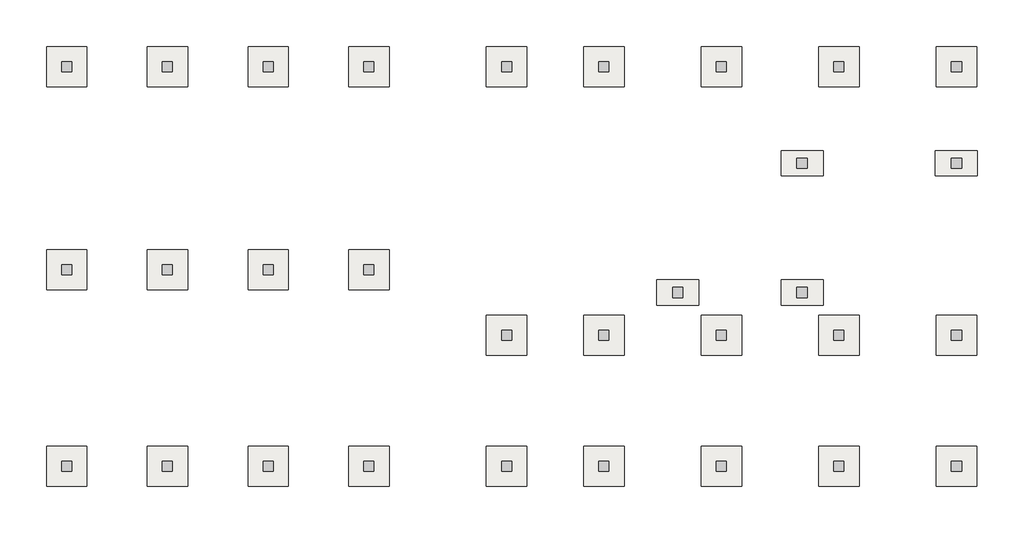
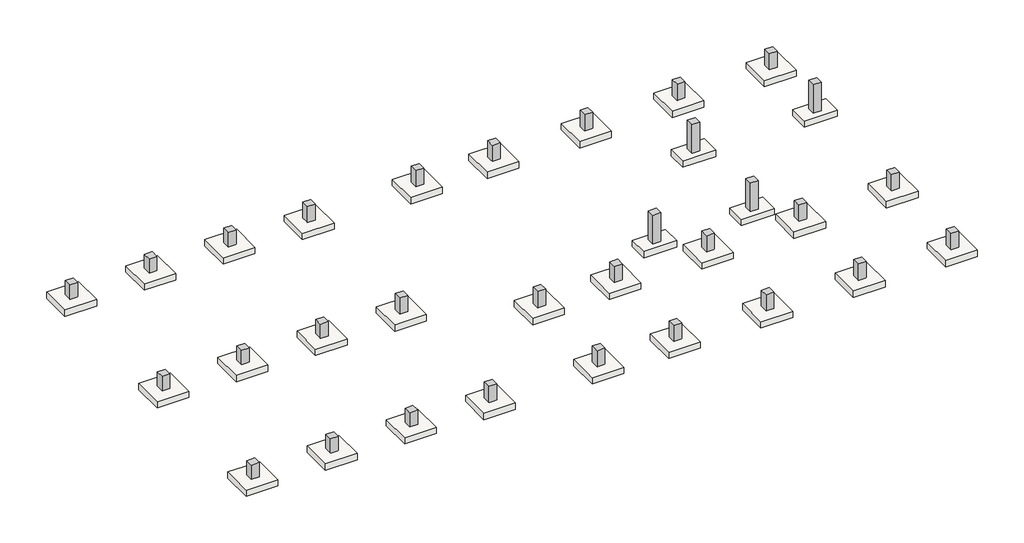
# Not in any storey: 31 columns, 31 slabs.
"""IFC4 building model written with IfcOpenShell, lengths in millimetres."""

import ifcopenshell
import ifcopenshell.guid

model = None  # the IFC model being written
_history = None  # IfcOwnerHistory: only IFC2X3 demands one
_inside = {}  # id of a spatial element -> (the spatial element, [elements in it])
_under = {}  # id of a project, library or spatial element -> (it, [spatial elements below it])
_declared = {}  # id of a project -> (the project, [libraries it declares])
_typed = {}  # id of a type object -> (the type object, [elements of that type])
_made_of = {}  # id of a material, layer set ... -> (it, [elements and type objects made of it])


def new_model(schema):
    """Start an empty IFC model of exactly this schema.

    Asked for "IFC4X3", IfcOpenShell would pick the latest addendum, in which some entities
    have other attributes; the version numbers below select the first issue.
    IFC2X3 requires an IfcOwnerHistory on every rooted entity: one is made here for all.
    """
    global model, _history
    if schema == "IFC4X3":
        model = ifcopenshell.file(schema_version=(4, 3, 0, 0))
    else:
        model = ifcopenshell.file(schema=schema)
    _inside.clear()
    _under.clear()
    _declared.clear()
    _typed.clear()
    _made_of.clear()
    _history = None
    if model.schema == "IFC2X3":
        org = make("IfcOrganization", Name="unknown")
        user = make(
            "IfcPersonAndOrganization",
            ThePerson=make("IfcPerson", FamilyName="unknown"),
            TheOrganization=org,
        )
        app = make(
            "IfcApplication",
            ApplicationDeveloper=org,
            Version="unknown",
            ApplicationFullName="unknown",
            ApplicationIdentifier="unknown",
        )
        _history = make(
            "IfcOwnerHistory",
            OwningUser=user,
            OwningApplication=app,
            ChangeAction="ADDED",
            CreationDate=0,
        )
    return model


def make(cls, **values):
    """One entity of the class cls with the attributes given. An attribute that is None is left unset."""
    return model.create_entity(
        cls, **{name: value for name, value in values.items() if value is not None}
    )


def rooted(cls, **values):
    """An entity with a GlobalId (a new one), such as an element, a storey or a relation."""
    return make(cls, GlobalId=ifcopenshell.guid.new(), OwnerHistory=_history, **values)


def si_unit(unit_type, name, prefix=None):
    """IfcSIUnit, for example si_unit("LENGTHUNIT", "METRE", prefix="MILLI")."""
    return make("IfcSIUnit", UnitType=unit_type, Prefix=prefix, Name=name)


def assignment(units):
    """IfcUnitAssignment: the units of a project."""
    return None if units is None else make("IfcUnitAssignment", Units=units)


def point(xyz):
    """IfcCartesianPoint."""
    return None if xyz is None else make("IfcCartesianPoint", Coordinates=xyz)


def direction(xyz):
    """IfcDirection."""
    return None if xyz is None else make("IfcDirection", DirectionRatios=xyz)


def frame(location, z_axis=None, x_axis=None):
    """IfcAxis2Placement3D, a coordinate frame: its origin and axes. An axis left out is left unset."""
    return make(
        "IfcAxis2Placement3D",
        Location=point(location),
        Axis=direction(z_axis),
        RefDirection=direction(x_axis),
    )


def origin():
    """The frame at (0, 0, 0) with its axes left unset."""
    return frame((0.0, 0.0, 0.0))


def place(relative_to, where):
    """IfcLocalPlacement: puts the frame where relative to a parent placement (None: the world)."""
    return make(
        "IfcLocalPlacement", PlacementRelTo=relative_to, RelativePlacement=where
    )


def context(
    kind, dimensions, precision=None, world=None, true_north=None, identifier=None
):
    """IfcGeometricRepresentationContext, for example the 3D "Model" context."""
    return make(
        "IfcGeometricRepresentationContext",
        ContextIdentifier=identifier,
        ContextType=kind,
        CoordinateSpaceDimension=dimensions,
        Precision=precision,
        WorldCoordinateSystem=world,
        TrueNorth=true_north,
    )


def project(units=None, contexts=None):
    """IfcProject with its units and contexts."""
    return rooted(
        "IfcProject",
        Name="project",
        RepresentationContexts=contexts,
        UnitsInContext=assignment(units),
    )


def spatial(cls, under=None, at=None, **own):
    """A site, building, storey or space (cls), placed at a placement, below another one or the project."""
    s = rooted(cls, ObjectPlacement=at, **own)
    if under is not None:
        _under.setdefault(under.id(), (under, []))[1].append(s)
    return s


def polyline(points):
    """IfcPolyline through the points."""
    return make("IfcPolyline", Points=[point(p) for p in points])


def outline(outer, holes=None, kind="AREA"):
    """IfcArbitraryClosedProfileDef: a profile drawn as a closed curve; with holes, ...WithVoids."""
    if holes is None:
        return make("IfcArbitraryClosedProfileDef", ProfileType=kind, OuterCurve=outer)
    return make(
        "IfcArbitraryProfileDefWithVoids",
        ProfileType=kind,
        OuterCurve=outer,
        InnerCurves=holes,
    )


def extrude(swept, where, along, depth):
    """IfcExtrudedAreaSolid: the profile swept, set in the frame where, extruded along a direction by depth."""
    return make(
        "IfcExtrudedAreaSolid",
        SweptArea=swept,
        Position=where,
        ExtrudedDirection=direction(along),
        Depth=depth,
    )


def shape(context_of_items, identifier, shape_type, items):
    """IfcShapeRepresentation: the items that make up one representation, for example the "Body"."""
    return make(
        "IfcShapeRepresentation",
        ContextOfItems=context_of_items,
        RepresentationIdentifier=identifier,
        RepresentationType=shape_type,
        Items=items,
    )


def source(mapping_origin, context_of_items, identifier, shape_type, items):
    """IfcRepresentationMap: a shape defined once, which mapped items show again and again."""
    return make(
        "IfcRepresentationMap",
        MappingOrigin=mapping_origin,
        MappedRepresentation=shape(context_of_items, identifier, shape_type, items),
    )


def transform(
    local_origin,
    x_axis=None,
    y_axis=None,
    z_axis=None,
    scale=None,
    scale2=None,
    scale3=None,
    uniform=True,
):
    """IfcCartesianTransformationOperator3D, or its non-uniform kind. x_axis, y_axis, z_axis: its Axis1, 2, 3."""
    if uniform:
        return make(
            "IfcCartesianTransformationOperator3D",
            Axis1=direction(x_axis),
            Axis2=direction(y_axis),
            LocalOrigin=point(local_origin),
            Scale=scale,
            Axis3=direction(z_axis),
        )
    return make(
        "IfcCartesianTransformationOperator3DnonUniform",
        Axis1=direction(x_axis),
        Axis2=direction(y_axis),
        LocalOrigin=point(local_origin),
        Scale=scale,
        Axis3=direction(z_axis),
        Scale2=scale2,
        Scale3=scale3,
    )


def mapped(mapping_source, mapping_target):
    """IfcMappedItem: shows the shape of a source again, moved by a transform."""
    return make(
        "IfcMappedItem", MappingSource=mapping_source, MappingTarget=mapping_target
    )


def made_of(thing, what):
    """Note that an element or type object is made of a material, layer set ...; save() writes the relation."""
    if what is not None:
        _made_of.setdefault(what.id(), (what, []))[1].append(thing)
    return thing


def element(
    cls,
    number,
    at=None,
    inside=None,
    cuts=None,
    type_object=None,
    material=None,
    context=None,
    identifier="Body",
    shape_type=None,
    held_by="IfcProductDefinitionShape",
    body=None,
    shapes=None,
    **own,
):
    """One element of the class cls, such as IfcWall. Its Tag is "e" and its number.

    at: its placement. inside: the storey or other place that contains it. cuts: it is an
    opening in that element (IfcRelVoidsElement). A single representation is given by context,
    identifier, shape_type and body (its items); several are given by shapes. held_by: the class
    of the entity that holds the representations. save() writes the other relations.
    """
    e = rooted(cls, Tag="e%d" % number, ObjectPlacement=at, **own)
    if body is not None:
        shapes = [shape(context, identifier, shape_type, body)]
    if shapes is not None:
        e.Representation = make(held_by, Representations=shapes)
    if inside is not None:
        _inside.setdefault(inside.id(), (inside, []))[1].append(e)
    if cuts is not None:
        rooted(
            "IfcRelVoidsElement", RelatingBuildingElement=cuts, RelatedOpeningElement=e
        )
    if type_object is not None:
        _typed.setdefault(type_object.id(), (type_object, []))[1].append(e)
    return made_of(e, material)


def aggregate(whole, parts):
    """IfcRelAggregates: a whole, such as a stair, and the parts it consists of."""
    return rooted("IfcRelAggregates", RelatingObject=whole, RelatedObjects=parts)


def save(model, path):
    """Write the relations noted so far, then the file.

    IfcRelAggregates (storeys below a building ...), IfcRelContainedInSpatialStructure (elements
    in a storey), IfcRelDefinesByType, IfcRelAssociatesMaterial and IfcRelDeclares: one each for
    every whole, place, type object, material and project.
    """
    for whole, parts in _under.values():
        aggregate(whole, parts)
    for where, things in _inside.values():
        rooted(
            "IfcRelContainedInSpatialStructure",
            RelatedElements=things,
            RelatingStructure=where,
        )
    for kind, things in _typed.values():
        rooted("IfcRelDefinesByType", RelatedObjects=things, RelatingType=kind)
    for what, things in _made_of.values():
        rooted("IfcRelAssociatesMaterial", RelatedObjects=things, RelatingMaterial=what)
    for by, libraries in _declared.values():
        rooted("IfcRelDeclares", RelatingContext=by, RelatedDefinitions=libraries)
    model.write(path)


def ft211_footing_rectangular_r1_5fe39465(model_context):
    return source(origin(), model_context, "Body", "SweptSolid", [
        extrude(outline(polyline([(1200.0, 1200.0), (1200.0, -1200.0), (-1200.0, -1200.0), (-1200.0, 1200.0), (1200.0, 1200.0)])), frame((0.0, 0.0, -500.0), z_axis=(0.0, 0.0, 1.0), x_axis=(1.0, 0.0, 0.0)), (0.0, 0.0, 1.0), 500.0),
    ])


def ft211_footing_rectangular_r1_907a7f09(model_context):
    return source(origin(), model_context, "Body", "SweptSolid", [
        extrude(outline(polyline([(1250.0, 750.0), (1250.0, -750.0), (-1250.0, -750.0), (-1250.0, 750.0), (1250.0, 750.0)])), frame((0.0, 0.0, -500.0), z_axis=(0.0, 0.0, 1.0), x_axis=(1.0, 0.0, 0.0)), (0.0, 0.0, 1.0), 500.0),
    ])


model = new_model("IFC4")

# Units and contexts
model_context = context("Model", 3, world=origin())
ifc_project = project(units=[si_unit("LENGTHUNIT", "METRE", prefix="MILLI")], contexts=[model_context])

# Site, building
site = spatial("IfcSite", under=ifc_project)
building = spatial("IfcBuilding", under=site)

# Columns
placement = place(None, origin())
element("IfcColumn", 1, ObjectType="RC_Column_Rectangular : H_SC_ACC_UG PED_W600xL600", at=placement, inside=building, context=model_context, shape_type="SweptSolid", body=[
    extrude(outline(polyline([(224.7, 12616.5208589), (224.7, 12016.5208589), (-375.3, 12016.5208589), (-375.3, 12616.5208589), (224.7, 12616.5208589)])), frame((0.0, 0.0, -1000.0), z_axis=(0.0, 0.0, 1.0), x_axis=(1.0, 0.0, 0.0)), (0.0, 0.0, 1.0), 1150.0),
])
element("IfcColumn", 2, ObjectType="RC_Column_Rectangular : H_SC_ACC_UG PED_W600xL600", at=placement, inside=building, context=model_context, shape_type="SweptSolid", body=[
    extrude(outline(polyline([(6224.7, 12616.5208589), (6224.7, 12016.5208589), (5624.7, 12016.5208589), (5624.7, 12616.5208589), (6224.7, 12616.5208589)])), frame((0.0, 0.0, -1000.0), z_axis=(0.0, 0.0, 1.0), x_axis=(1.0, 0.0, 0.0)), (0.0, 0.0, 1.0), 1150.0),
])
element("IfcColumn", 3, ObjectType="RC_Column_Rectangular : H_SC_ACC_UG PED_W600xL600", at=placement, inside=building, context=model_context, shape_type="SweptSolid", body=[
    extrude(outline(polyline([(12224.7, 12616.5208589), (12224.7, 12016.5208589), (11624.7, 12016.5208589), (11624.7, 12616.5208589), (12224.7, 12616.5208589)])), frame((0.0, 0.0, -1000.0), z_axis=(0.0, 0.0, 1.0), x_axis=(1.0, 0.0, 0.0)), (0.0, 0.0, 1.0), 1150.0),
])
element("IfcColumn", 4, ObjectType="RC_Column_Rectangular : H_SC_ACC_UG PED_W600xL600", at=placement, inside=building, context=model_context, shape_type="SweptSolid", body=[
    extrude(outline(polyline([(18224.7, 12616.5208589), (18224.7, 12016.5208589), (17624.7, 12016.5208589), (17624.7, 12616.5208589), (18224.7, 12616.5208589)])), frame((0.0, 0.0, -1150.0), z_axis=(0.0, 0.0, 1.0), x_axis=(1.0, 0.0, 0.0)), (0.0, 0.0, 1.0), 1300.0),
])
element("IfcColumn", 5, ObjectType="RC_Column_Rectangular : H_SC_ACC_UG PED_W600xL600", at=placement, inside=building, context=model_context, shape_type="SweptSolid", body=[
    extrude(outline(polyline([(224.7, 24716.5208589), (224.7, 24116.5208589), (-375.3, 24116.5208589), (-375.3, 24716.5208589), (224.7, 24716.5208589)])), frame((0.0, 0.0, -1000.0), z_axis=(0.0, 0.0, 1.0), x_axis=(1.0, 0.0, 0.0)), (0.0, 0.0, 1.0), 1150.0),
])
element("IfcColumn", 6, ObjectType="RC_Column_Rectangular : H_SC_ACC_UG PED_W600xL600", at=placement, inside=building, context=model_context, shape_type="SweptSolid", body=[
    extrude(outline(polyline([(6224.7, 24716.5208589), (6224.7, 24116.5208589), (5624.7, 24116.5208589), (5624.7, 24716.5208589), (6224.7, 24716.5208589)])), frame((0.0, 0.0, -1000.0), z_axis=(0.0, 0.0, 1.0), x_axis=(1.0, 0.0, 0.0)), (0.0, 0.0, 1.0), 1150.0),
])
element("IfcColumn", 7, ObjectType="RC_Column_Rectangular : H_SC_ACC_UG PED_W600xL600", at=placement, inside=building, context=model_context, shape_type="SweptSolid", body=[
    extrude(outline(polyline([(12224.7, 24716.5208589), (12224.7, 24116.5208589), (11624.7, 24116.5208589), (11624.7, 24716.5208589), (12224.7, 24716.5208589)])), frame((0.0, 0.0, -1000.0), z_axis=(0.0, 0.0, 1.0), x_axis=(1.0, 0.0, 0.0)), (0.0, 0.0, 1.0), 1150.0),
])
element("IfcColumn", 8, ObjectType="RC_Column_Rectangular : H_SC_ACC_UG PED_W600xL600", at=placement, inside=building, context=model_context, shape_type="SweptSolid", body=[
    extrude(outline(polyline([(18224.7, 24716.5208589), (18224.7, 24116.5208589), (17624.7, 24116.5208589), (17624.7, 24716.5208589), (18224.7, 24716.5208589)])), frame((0.0, 0.0, -1150.0), z_axis=(0.0, 0.0, 1.0), x_axis=(1.0, 0.0, 0.0)), (0.0, 0.0, 1.0), 1300.0),
])
element("IfcColumn", 9, ObjectType="RC_Column_Rectangular : H_SC_ACC_UG PED_W600xL600", at=placement, inside=building, context=model_context, shape_type="SweptSolid", body=[
    extrude(outline(polyline([(26424.7, 24716.5208589), (26424.7, 24116.5208589), (25824.7, 24116.5208589), (25824.7, 24716.5208589), (26424.7, 24716.5208589)])), frame((0.0, 0.0, -1150.0), z_axis=(0.0, 0.0, 1.0), x_axis=(1.0, 0.0, 0.0)), (0.0, 0.0, 1.0), 1300.0),
])
element("IfcColumn", 10, ObjectType="RC_Column_Rectangular : H_SC_ACC_UG PED_W600xL600", at=placement, inside=building, context=model_context, shape_type="SweptSolid", body=[
    extrude(outline(polyline([(32224.7, 24716.5208589), (32224.7, 24116.5208589), (31624.7, 24116.5208589), (31624.7, 24716.5208589), (32224.7, 24716.5208589)])), frame((0.0, 0.0, -1150.0), z_axis=(0.0, 0.0, 1.0), x_axis=(1.0, 0.0, 0.0)), (0.0, 0.0, 1.0), 1300.0),
])
element("IfcColumn", 11, ObjectType="RC_Column_Rectangular : H_SC_ACC_UG PED_W600xL600", at=placement, inside=building, context=model_context, shape_type="SweptSolid", body=[
    extrude(outline(polyline([(39224.7, 24716.5208589), (39224.7, 24116.5208589), (38624.7, 24116.5208589), (38624.7, 24716.5208589), (39224.7, 24716.5208589)])), frame((0.0, 0.0, -1150.0), z_axis=(0.0, 0.0, 1.0), x_axis=(1.0, 0.0, 0.0)), (0.0, 0.0, 1.0), 1300.0),
])
element("IfcColumn", 12, ObjectType="RC_Column_Rectangular : H_SC_ACC_UG PED_W600xL600", at=placement, inside=building, context=model_context, shape_type="SweptSolid", body=[
    extrude(outline(polyline([(46224.7, 24716.5208589), (46224.7, 24116.5208589), (45624.7, 24116.5208589), (45624.7, 24716.5208589), (46224.7, 24716.5208589)])), frame((0.0, 0.0, -1150.0), z_axis=(0.0, 0.0, 1.0), x_axis=(1.0, 0.0, 0.0)), (0.0, 0.0, 1.0), 1300.0),
])
element("IfcColumn", 13, ObjectType="RC_Column_Rectangular : H_SC_ACC_UG PED_W600xL600", at=placement, inside=building, context=model_context, shape_type="SweptSolid", body=[
    extrude(outline(polyline([(53224.7, 24716.5208589), (53224.7, 24116.5208589), (52624.7, 24116.5208589), (52624.7, 24716.5208589), (53224.7, 24716.5208589)])), frame((0.0, 0.0, -1150.0), z_axis=(0.0, 0.0, 1.0), x_axis=(1.0, 0.0, 0.0)), (0.0, 0.0, 1.0), 1300.0),
])
element("IfcColumn", 14, ObjectType="RC_Column_Rectangular : H_SC_ACC_UG PED_W600xL600", at=placement, inside=building, context=model_context, shape_type="SweptSolid", body=[
    extrude(outline(polyline([(26424.7, 8716.5208589), (26424.7, 8116.5208589), (25824.7, 8116.5208589), (25824.7, 8716.5208589), (26424.7, 8716.5208589)])), frame((0.0, 0.0, -1150.0), z_axis=(0.0, 0.0, 1.0), x_axis=(1.0, 0.0, 0.0)), (0.0, 0.0, 1.0), 1300.0),
])
element("IfcColumn", 15, ObjectType="RC_Column_Rectangular : H_SC_ACC_UG PED_W600xL600", at=placement, inside=building, context=model_context, shape_type="SweptSolid", body=[
    extrude(outline(polyline([(32224.7, 8716.5208589), (32224.7, 8116.5208589), (31624.7, 8116.5208589), (31624.7, 8716.5208589), (32224.7, 8716.5208589)])), frame((0.0, 0.0, -1150.0), z_axis=(0.0, 0.0, 1.0), x_axis=(1.0, 0.0, 0.0)), (0.0, 0.0, 1.0), 1300.0),
])
element("IfcColumn", 16, ObjectType="RC_Column_Rectangular : H_SC_ACC_UG PED_W600xL600", at=placement, inside=building, context=model_context, shape_type="SweptSolid", body=[
    extrude(outline(polyline([(39224.7, 8716.5208589), (39224.7, 8116.5208589), (38624.7, 8116.5208589), (38624.7, 8716.5208589), (39224.7, 8716.5208589)])), frame((0.0, 0.0, -1150.0), z_axis=(0.0, 0.0, 1.0), x_axis=(1.0, 0.0, 0.0)), (0.0, 0.0, 1.0), 1300.0),
])
element("IfcColumn", 17, ObjectType="RC_Column_Rectangular : H_SC_ACC_UG PED_W600xL600", at=placement, inside=building, context=model_context, shape_type="SweptSolid", body=[
    extrude(outline(polyline([(46224.7, 8716.5208589), (46224.7, 8116.5208589), (45624.7, 8116.5208589), (45624.7, 8716.5208589), (46224.7, 8716.5208589)])), frame((0.0, 0.0, -1150.0), z_axis=(0.0, 0.0, 1.0), x_axis=(1.0, 0.0, 0.0)), (0.0, 0.0, 1.0), 1300.0),
])
element("IfcColumn", 18, ObjectType="RC_Column_Rectangular : H_SC_ACC_UG PED_W600xL600", at=placement, inside=building, context=model_context, shape_type="SweptSolid", body=[
    extrude(outline(polyline([(53224.7, 8716.5208589), (53224.7, 8116.5208589), (52624.7, 8116.5208589), (52624.7, 8716.5208589), (53224.7, 8716.5208589)])), frame((0.0, 0.0, -1150.0), z_axis=(0.0, 0.0, 1.0), x_axis=(1.0, 0.0, 0.0)), (0.0, 0.0, 1.0), 1300.0),
])
element("IfcColumn", 19, ObjectType="RC_Column_Rectangular : H_SC_ACC_UG PED_W600xL600", at=placement, inside=building, context=model_context, shape_type="SweptSolid", body=[
    extrude(outline(polyline([(224.7, 916.5208589), (224.7, 316.5208589), (-375.3, 316.5208589), (-375.3, 916.5208589), (224.7, 916.5208589)])), frame((0.0, 0.0, -1000.0), z_axis=(0.0, 0.0, 1.0), x_axis=(1.0, 0.0, 0.0)), (0.0, 0.0, 1.0), 1150.0),
])
element("IfcColumn", 20, ObjectType="RC_Column_Rectangular : H_SC_ACC_UG PED_W600xL600", at=placement, inside=building, context=model_context, shape_type="SweptSolid", body=[
    extrude(outline(polyline([(6224.7, 916.5208589), (6224.7, 316.5208589), (5624.7, 316.5208589), (5624.7, 916.5208589), (6224.7, 916.5208589)])), frame((0.0, 0.0, -1000.0), z_axis=(0.0, 0.0, 1.0), x_axis=(1.0, 0.0, 0.0)), (0.0, 0.0, 1.0), 1150.0),
])
element("IfcColumn", 21, ObjectType="RC_Column_Rectangular : H_SC_ACC_UG PED_W600xL600", at=placement, inside=building, context=model_context, shape_type="SweptSolid", body=[
    extrude(outline(polyline([(12224.7, 916.5208589), (12224.7, 316.5208589), (11624.7, 316.5208589), (11624.7, 916.5208589), (12224.7, 916.5208589)])), frame((0.0, 0.0, -1000.0), z_axis=(0.0, 0.0, 1.0), x_axis=(1.0, 0.0, 0.0)), (0.0, 0.0, 1.0), 1150.0),
])
element("IfcColumn", 22, ObjectType="RC_Column_Rectangular : H_SC_ACC_UG PED_W600xL600", at=placement, inside=building, context=model_context, shape_type="SweptSolid", body=[
    extrude(outline(polyline([(18224.7, 916.5208589), (18224.7, 316.5208589), (17624.7, 316.5208589), (17624.7, 916.5208589), (18224.7, 916.5208589)])), frame((0.0, 0.0, -1150.0), z_axis=(0.0, 0.0, 1.0), x_axis=(1.0, 0.0, 0.0)), (0.0, 0.0, 1.0), 1300.0),
])
element("IfcColumn", 23, ObjectType="RC_Column_Rectangular : H_SC_ACC_UG PED_W600xL600", at=placement, inside=building, context=model_context, shape_type="SweptSolid", body=[
    extrude(outline(polyline([(26424.7, 916.5208589), (26424.7, 316.5208589), (25824.7, 316.5208589), (25824.7, 916.5208589), (26424.7, 916.5208589)])), frame((0.0, 0.0, -1150.0), z_axis=(0.0, 0.0, 1.0), x_axis=(1.0, 0.0, 0.0)), (0.0, 0.0, 1.0), 1300.0),
])
element("IfcColumn", 24, ObjectType="RC_Column_Rectangular : H_SC_ACC_UG PED_W600xL600", at=placement, inside=building, context=model_context, shape_type="SweptSolid", body=[
    extrude(outline(polyline([(32224.7, 916.5208589), (32224.7, 316.5208589), (31624.7, 316.5208589), (31624.7, 916.5208589), (32224.7, 916.5208589)])), frame((0.0, 0.0, -1150.0), z_axis=(0.0, 0.0, 1.0), x_axis=(1.0, 0.0, 0.0)), (0.0, 0.0, 1.0), 1300.0),
])
element("IfcColumn", 25, ObjectType="RC_Column_Rectangular : H_SC_ACC_UG PED_W600xL600", at=placement, inside=building, context=model_context, shape_type="SweptSolid", body=[
    extrude(outline(polyline([(39224.7, 916.5208589), (39224.7, 316.5208589), (38624.7, 316.5208589), (38624.7, 916.5208589), (39224.7, 916.5208589)])), frame((0.0, 0.0, -1150.0), z_axis=(0.0, 0.0, 1.0), x_axis=(1.0, 0.0, 0.0)), (0.0, 0.0, 1.0), 1300.0),
])
element("IfcColumn", 26, ObjectType="RC_Column_Rectangular : H_SC_ACC_UG PED_W600xL600", at=placement, inside=building, context=model_context, shape_type="SweptSolid", body=[
    extrude(outline(polyline([(46224.7, 916.5208589), (46224.7, 316.5208589), (45624.7, 316.5208589), (45624.7, 916.5208589), (46224.7, 916.5208589)])), frame((0.0, 0.0, -1150.0), z_axis=(0.0, 0.0, 1.0), x_axis=(1.0, 0.0, 0.0)), (0.0, 0.0, 1.0), 1300.0),
])
element("IfcColumn", 27, ObjectType="RC_Column_Rectangular : H_SC_ACC_UG PED_W600xL600", at=placement, inside=building, context=model_context, shape_type="SweptSolid", body=[
    extrude(outline(polyline([(53224.7, 916.5208589), (53224.7, 316.5208589), (52624.7, 316.5208589), (52624.7, 916.5208589), (53224.7, 916.5208589)])), frame((0.0, 0.0, -1150.0), z_axis=(0.0, 0.0, 1.0), x_axis=(1.0, 0.0, 0.0)), (0.0, 0.0, 1.0), 1300.0),
])
element("IfcColumn", 28, ObjectType="RC_Column_Rectangular : H_SC_ACC_UG PED_W600xL600", at=placement, inside=building, context=model_context, shape_type="SweptSolid", body=[
    extrude(outline(polyline([(36624.7, 11266.5208589), (36624.7, 10666.5208589), (36024.7, 10666.5208589), (36024.7, 11266.5208589), (36624.7, 11266.5208589)])), frame((0.0, 0.0, -1150.0), z_axis=(0.0, 0.0, 1.0), x_axis=(1.0, 0.0, 0.0)), (0.0, 0.0, 1.0), 2300.0),
])
element("IfcColumn", 29, ObjectType="RC_Column_Rectangular : H_SC_ACC_UG PED_W600xL600", at=placement, inside=building, context=model_context, shape_type="SweptSolid", body=[
    extrude(outline(polyline([(44024.7, 11266.5208589), (44024.7, 10666.5208589), (43424.7, 10666.5208589), (43424.7, 11266.5208589), (44024.7, 11266.5208589)])), frame((0.0, 0.0, -1150.0), z_axis=(0.0, 0.0, 1.0), x_axis=(1.0, 0.0, 0.0)), (0.0, 0.0, 1.0), 2300.0),
])
element("IfcColumn", 30, ObjectType="RC_Column_Rectangular : H_SC_ACC_UG PED_W600xL600", at=placement, inside=building, context=model_context, shape_type="SweptSolid", body=[
    extrude(outline(polyline([(44024.7, 18966.5208589), (44024.7, 18366.5208589), (43424.7, 18366.5208589), (43424.7, 18966.5208589), (44024.7, 18966.5208589)])), frame((0.0, 0.0, -1150.0), z_axis=(0.0, 0.0, 1.0), x_axis=(1.0, 0.0, 0.0)), (0.0, 0.0, 1.0), 2300.0),
])
element("IfcColumn", 31, ObjectType="RC_Column_Rectangular : H_SC_ACC_UG PED_W600xL600", at=placement, inside=building, context=model_context, shape_type="SweptSolid", body=[
    extrude(outline(polyline([(53224.7, 18966.5208589), (53224.7, 18366.5208589), (52624.7, 18366.5208589), (52624.7, 18966.5208589), (53224.7, 18966.5208589)])), frame((0.0, 0.0, -1150.0), z_axis=(0.0, 0.0, 1.0), x_axis=(1.0, 0.0, 0.0)), (0.0, 0.0, 1.0), 2300.0),
])

# Slabs
ft211_footing_rectangular_r1_shape = ft211_footing_rectangular_r1_5fe39465(model_context)
element("IfcSlab", 32, ObjectType="FT211-Footing-Rectangular_R1 : H_SF_ACF_W2400xL2400xT500_Bitumen", at=placement, inside=building, context=model_context, shape_type="MappedRepresentation", body=[
    mapped(ft211_footing_rectangular_r1_shape, transform((-75.3, 12316.5208589, -1000.0), x_axis=(1.0, 0.0, 0.0), y_axis=(0.0, 1.0, 0.0), z_axis=(0.0, 0.0, 1.0))),
])
element("IfcSlab", 33, ObjectType="FT211-Footing-Rectangular_R1 : H_SF_ACF_W2400xL2400xT500_Bitumen", at=placement, inside=building, context=model_context, shape_type="MappedRepresentation", body=[
    mapped(ft211_footing_rectangular_r1_shape, transform((5924.7, 12316.5208589, -1000.0), x_axis=(1.0, 0.0, 0.0), y_axis=(0.0, 1.0, 0.0), z_axis=(0.0, 0.0, 1.0))),
])
element("IfcSlab", 34, ObjectType="FT211-Footing-Rectangular_R1 : H_SF_ACF_W2400xL2400xT500_Bitumen", at=placement, inside=building, context=model_context, shape_type="MappedRepresentation", body=[
    mapped(ft211_footing_rectangular_r1_shape, transform((11924.7, 12316.5208589, -1000.0), x_axis=(1.0, 0.0, 0.0), y_axis=(0.0, 1.0, 0.0), z_axis=(0.0, 0.0, 1.0))),
])
element("IfcSlab", 35, ObjectType="FT211-Footing-Rectangular_R1 : H_SF_ACF_W2400xL2400xT500_Bitumen", at=placement, inside=building, context=model_context, shape_type="MappedRepresentation", body=[
    mapped(ft211_footing_rectangular_r1_shape, transform((17924.7, 12316.5208589, -1150.0), x_axis=(1.0, 0.0, 0.0), y_axis=(0.0, 1.0, 0.0), z_axis=(0.0, 0.0, 1.0))),
])
element("IfcSlab", 36, ObjectType="FT211-Footing-Rectangular_R1 : H_SF_ACF_W2400xL2400xT500_Bitumen", at=placement, inside=building, context=model_context, shape_type="MappedRepresentation", body=[
    mapped(ft211_footing_rectangular_r1_shape, transform((-75.3, 24416.5208589, -1000.0), x_axis=(1.0, 0.0, 0.0), y_axis=(0.0, 1.0, 0.0), z_axis=(0.0, 0.0, 1.0))),
])
element("IfcSlab", 37, ObjectType="FT211-Footing-Rectangular_R1 : H_SF_ACF_W2400xL2400xT500_Bitumen", at=placement, inside=building, context=model_context, shape_type="MappedRepresentation", body=[
    mapped(ft211_footing_rectangular_r1_shape, transform((5924.7, 24416.5208589, -1000.0), x_axis=(1.0, 0.0, 0.0), y_axis=(0.0, 1.0, 0.0), z_axis=(0.0, 0.0, 1.0))),
])
element("IfcSlab", 38, ObjectType="FT211-Footing-Rectangular_R1 : H_SF_ACF_W2400xL2400xT500_Bitumen", at=placement, inside=building, context=model_context, shape_type="MappedRepresentation", body=[
    mapped(ft211_footing_rectangular_r1_shape, transform((11924.7, 24416.5208589, -1000.0), x_axis=(1.0, 0.0, 0.0), y_axis=(0.0, 1.0, 0.0), z_axis=(0.0, 0.0, 1.0))),
])
element("IfcSlab", 39, ObjectType="FT211-Footing-Rectangular_R1 : H_SF_ACF_W2400xL2400xT500_Bitumen", at=placement, inside=building, context=model_context, shape_type="MappedRepresentation", body=[
    mapped(ft211_footing_rectangular_r1_shape, transform((17924.7, 24416.5208589, -1150.0), x_axis=(1.0, 0.0, 0.0), y_axis=(0.0, 1.0, 0.0), z_axis=(0.0, 0.0, 1.0))),
])
element("IfcSlab", 40, ObjectType="FT211-Footing-Rectangular_R1 : H_SF_ACF_W2400xL2400xT500_Bitumen", at=placement, inside=building, context=model_context, shape_type="MappedRepresentation", body=[
    mapped(ft211_footing_rectangular_r1_shape, transform((26124.7, 24416.5208589, -1150.0), x_axis=(1.0, 0.0, 0.0), y_axis=(0.0, 1.0, 0.0), z_axis=(0.0, 0.0, 1.0))),
])
element("IfcSlab", 41, ObjectType="FT211-Footing-Rectangular_R1 : H_SF_ACF_W2400xL2400xT500_Bitumen", at=placement, inside=building, context=model_context, shape_type="MappedRepresentation", body=[
    mapped(ft211_footing_rectangular_r1_shape, transform((31924.7, 24416.5208589, -1150.0), x_axis=(1.0, 0.0, 0.0), y_axis=(0.0, 1.0, 0.0), z_axis=(0.0, 0.0, 1.0))),
])
element("IfcSlab", 42, ObjectType="FT211-Footing-Rectangular_R1 : H_SF_ACF_W2400xL2400xT500_Bitumen", at=placement, inside=building, context=model_context, shape_type="MappedRepresentation", body=[
    mapped(ft211_footing_rectangular_r1_shape, transform((38924.7, 24416.5208589, -1150.0), x_axis=(1.0, 0.0, 0.0), y_axis=(0.0, 1.0, 0.0), z_axis=(0.0, 0.0, 1.0))),
])
element("IfcSlab", 43, ObjectType="FT211-Footing-Rectangular_R1 : H_SF_ACF_W2400xL2400xT500_Bitumen", at=placement, inside=building, context=model_context, shape_type="MappedRepresentation", body=[
    mapped(ft211_footing_rectangular_r1_shape, transform((45924.7, 24416.5208589, -1150.0), x_axis=(1.0, 0.0, 0.0), y_axis=(0.0, 1.0, 0.0), z_axis=(0.0, 0.0, 1.0))),
])
element("IfcSlab", 44, ObjectType="FT211-Footing-Rectangular_R1 : H_SF_ACF_W2400xL2400xT500_Bitumen", at=placement, inside=building, context=model_context, shape_type="MappedRepresentation", body=[
    mapped(ft211_footing_rectangular_r1_shape, transform((52924.7, 24416.5208589, -1150.0), x_axis=(1.0, 0.0, 0.0), y_axis=(0.0, 1.0, 0.0), z_axis=(0.0, 0.0, 1.0))),
])
element("IfcSlab", 45, ObjectType="FT211-Footing-Rectangular_R1 : H_SF_ACF_W2400xL2400xT500_Bitumen", at=placement, inside=building, context=model_context, shape_type="MappedRepresentation", body=[
    mapped(ft211_footing_rectangular_r1_shape, transform((26124.7, 8416.5208589, -1150.0), x_axis=(1.0, 0.0, 0.0), y_axis=(0.0, 1.0, 0.0), z_axis=(0.0, 0.0, 1.0))),
])
element("IfcSlab", 46, ObjectType="FT211-Footing-Rectangular_R1 : H_SF_ACF_W2400xL2400xT500_Bitumen", at=placement, inside=building, context=model_context, shape_type="MappedRepresentation", body=[
    mapped(ft211_footing_rectangular_r1_shape, transform((31924.7, 8416.5208589, -1150.0), x_axis=(1.0, 0.0, 0.0), y_axis=(0.0, 1.0, 0.0), z_axis=(0.0, 0.0, 1.0))),
])
element("IfcSlab", 47, ObjectType="FT211-Footing-Rectangular_R1 : H_SF_ACF_W2400xL2400xT500_Bitumen", at=placement, inside=building, context=model_context, shape_type="MappedRepresentation", body=[
    mapped(ft211_footing_rectangular_r1_shape, transform((38924.7, 8416.5208589, -1150.0), x_axis=(1.0, 0.0, 0.0), y_axis=(0.0, 1.0, 0.0), z_axis=(0.0, 0.0, 1.0))),
])
element("IfcSlab", 48, ObjectType="FT211-Footing-Rectangular_R1 : H_SF_ACF_W2400xL2400xT500_Bitumen", at=placement, inside=building, context=model_context, shape_type="MappedRepresentation", body=[
    mapped(ft211_footing_rectangular_r1_shape, transform((45924.7, 8416.5208589, -1150.0), x_axis=(1.0, 0.0, 0.0), y_axis=(0.0, 1.0, 0.0), z_axis=(0.0, 0.0, 1.0))),
])
element("IfcSlab", 49, ObjectType="FT211-Footing-Rectangular_R1 : H_SF_ACF_W2400xL2400xT500_Bitumen", at=placement, inside=building, context=model_context, shape_type="MappedRepresentation", body=[
    mapped(ft211_footing_rectangular_r1_shape, transform((52924.7, 8416.5208589, -1150.0), x_axis=(1.0, 0.0, 0.0), y_axis=(0.0, 1.0, 0.0), z_axis=(0.0, 0.0, 1.0))),
])
element("IfcSlab", 50, ObjectType="FT211-Footing-Rectangular_R1 : H_SF_ACF_W2400xL2400xT500_Bitumen", at=placement, inside=building, context=model_context, shape_type="MappedRepresentation", body=[
    mapped(ft211_footing_rectangular_r1_shape, transform((-75.3, 616.5208589, -1000.0), x_axis=(1.0, 0.0, 0.0), y_axis=(0.0, 1.0, 0.0), z_axis=(0.0, 0.0, 1.0))),
])
element("IfcSlab", 51, ObjectType="FT211-Footing-Rectangular_R1 : H_SF_ACF_W2400xL2400xT500_Bitumen", at=placement, inside=building, context=model_context, shape_type="MappedRepresentation", body=[
    mapped(ft211_footing_rectangular_r1_shape, transform((5924.7, 616.5208589, -1000.0), x_axis=(1.0, 0.0, 0.0), y_axis=(0.0, 1.0, 0.0), z_axis=(0.0, 0.0, 1.0))),
])
element("IfcSlab", 52, ObjectType="FT211-Footing-Rectangular_R1 : H_SF_ACF_W2400xL2400xT500_Bitumen", at=placement, inside=building, context=model_context, shape_type="MappedRepresentation", body=[
    mapped(ft211_footing_rectangular_r1_shape, transform((11924.7, 616.5208589, -1000.0), x_axis=(1.0, 0.0, 0.0), y_axis=(0.0, 1.0, 0.0), z_axis=(0.0, 0.0, 1.0))),
])
element("IfcSlab", 53, ObjectType="FT211-Footing-Rectangular_R1 : H_SF_ACF_W2400xL2400xT500_Bitumen", at=placement, inside=building, context=model_context, shape_type="MappedRepresentation", body=[
    mapped(ft211_footing_rectangular_r1_shape, transform((17924.7, 616.5208589, -1150.0), x_axis=(1.0, 0.0, 0.0), y_axis=(0.0, 1.0, 0.0), z_axis=(0.0, 0.0, 1.0))),
])
element("IfcSlab", 54, ObjectType="FT211-Footing-Rectangular_R1 : H_SF_ACF_W2400xL2400xT500_Bitumen", at=placement, inside=building, context=model_context, shape_type="MappedRepresentation", body=[
    mapped(ft211_footing_rectangular_r1_shape, transform((26124.7, 616.5208589, -1150.0), x_axis=(1.0, 0.0, 0.0), y_axis=(0.0, 1.0, 0.0), z_axis=(0.0, 0.0, 1.0))),
])
element("IfcSlab", 55, ObjectType="FT211-Footing-Rectangular_R1 : H_SF_ACF_W2400xL2400xT500_Bitumen", at=placement, inside=building, context=model_context, shape_type="MappedRepresentation", body=[
    mapped(ft211_footing_rectangular_r1_shape, transform((31924.7, 616.5208589, -1150.0), x_axis=(1.0, 0.0, 0.0), y_axis=(0.0, 1.0, 0.0), z_axis=(0.0, 0.0, 1.0))),
])
element("IfcSlab", 56, ObjectType="FT211-Footing-Rectangular_R1 : H_SF_ACF_W2400xL2400xT500_Bitumen", at=placement, inside=building, context=model_context, shape_type="MappedRepresentation", body=[
    mapped(ft211_footing_rectangular_r1_shape, transform((38924.7, 616.5208589, -1150.0), x_axis=(1.0, 0.0, 0.0), y_axis=(0.0, 1.0, 0.0), z_axis=(0.0, 0.0, 1.0))),
])
element("IfcSlab", 57, ObjectType="FT211-Footing-Rectangular_R1 : H_SF_ACF_W2400xL2400xT500_Bitumen", at=placement, inside=building, context=model_context, shape_type="MappedRepresentation", body=[
    mapped(ft211_footing_rectangular_r1_shape, transform((45924.7, 616.5208589, -1150.0), x_axis=(1.0, 0.0, 0.0), y_axis=(0.0, 1.0, 0.0), z_axis=(0.0, 0.0, 1.0))),
])
element("IfcSlab", 58, ObjectType="FT211-Footing-Rectangular_R1 : H_SF_ACF_W2400xL2400xT500_Bitumen", at=placement, inside=building, context=model_context, shape_type="MappedRepresentation", body=[
    mapped(ft211_footing_rectangular_r1_shape, transform((52924.7, 616.5208589, -1150.0), x_axis=(1.0, 0.0, 0.0), y_axis=(0.0, 1.0, 0.0), z_axis=(0.0, 0.0, 1.0))),
])
ft211_footing_rectangular_r1_2_shape = ft211_footing_rectangular_r1_907a7f09(model_context)
element("IfcSlab", 59, ObjectType="FT211-Footing-Rectangular_R1 : H_SF_ACF_W2500xL1500xT500_Bitumen", at=placement, inside=building, context=model_context, shape_type="MappedRepresentation", body=[
    mapped(ft211_footing_rectangular_r1_2_shape, transform((36324.7, 10966.5208589, -1150.0), x_axis=(1.0, 0.0, 0.0), y_axis=(0.0, 1.0, 0.0), z_axis=(0.0, 0.0, 1.0))),
])
element("IfcSlab", 60, ObjectType="FT211-Footing-Rectangular_R1 : H_SF_ACF_W2500xL1500xT500_Bitumen", at=placement, inside=building, context=model_context, shape_type="MappedRepresentation", body=[
    mapped(ft211_footing_rectangular_r1_2_shape, transform((43724.7, 10966.5208589, -1150.0), x_axis=(1.0, 0.0, 0.0), y_axis=(0.0, 1.0, 0.0), z_axis=(0.0, 0.0, 1.0))),
])
element("IfcSlab", 61, ObjectType="FT211-Footing-Rectangular_R1 : H_SF_ACF_W2500xL1500xT500_Bitumen", at=placement, inside=building, context=model_context, shape_type="MappedRepresentation", body=[
    mapped(ft211_footing_rectangular_r1_2_shape, transform((43724.7, 18666.5208589, -1150.0), x_axis=(1.0, 0.0, 0.0), y_axis=(0.0, 1.0, 0.0), z_axis=(0.0, 0.0, 1.0))),
])
element("IfcSlab", 62, ObjectType="FT211-Footing-Rectangular_R1 : H_SF_ACF_W2500xL1500xT500_Bitumen", at=placement, inside=building, context=model_context, shape_type="MappedRepresentation", body=[
    mapped(ft211_footing_rectangular_r1_2_shape, transform((52924.7, 18666.5208589, -1150.0), x_axis=(1.0, 0.0, 0.0), y_axis=(0.0, 1.0, 0.0), z_axis=(0.0, 0.0, 1.0))),
])

save(model, "model.ifc")

# Revit data of these elements
# Type "RC_Column_Rectangular : H_SC_ACC_UG PED_W600xL600"
#   Width = 0.600 m
#   Length = 0.600 m
#   hec_material3 [instance default] = none
#   hec_material2 [instance default] = none
#   hec_material1 [instance default] = none
#   Structural Material [instance default] = none
#   Description = (empty or 0)
# Type "FT211-Footing-Rectangular_R1 : H_SF_ACF_W2400xL2400xT500_Bitumen"
#   Top bar = "D25@300"
#   Description = "UG Shallow Foundation"
#   Bottom bar = "D20@300"
#   Width = 2.400 m
#   Length = 2.400 m
#   Foundation Thickness = 0.500 m
#   Structural Material [instance default] = none
#   Assembly Code = ""
# Type "FT211-Footing-Rectangular_R1 : H_SF_ACF_W2500xL1500xT500_Bitumen"
#   Top bar = "D25@300"
#   Description = "UG Shallow Foundation"
#   Bottom bar = "D20@300"
#   Width = 2.500 m
#   Length = 1.500 m
#   Foundation Thickness = 0.500 m
#   Structural Material [instance default] = none
#   Assembly Code = ""
# Elements 1, 2, 3, 4, 5, 6, 7, 8, 9, 10, 11, 12, 13, 14, 15, 16, 17, 18, 19, 20, 21, 22, 23, 24, 25, 26, 27, 28, 29, 30, 31 (IfcColumn, "RC_Column_Rectangular : H_SC_ACC_UG PED_W600xL600")
#   Comments = ""
#   hec_material3 = none
#   hec_material2 = none
#   hec_material1 = none
#   Structural Material = none
#   Phase Created = New Construction
# Elements 32, 33, 34, 35, 36, 37, 38, 39, 40, 41, 42, 43, 44, 45, 46, 47, 48, 49, 50, 51, 52, 53, 54, 55, 56, 57, 58 (IfcSlab, "FT211-Footing-Rectangular_R1 : H_SF_ACF_W2400xL2400xT500_Bitumen")
#   Comments = ""
#   Structural Material = none
#   Phase Created = New Construction
# Elements 59, 60, 61, 62 (IfcSlab, "FT211-Footing-Rectangular_R1 : H_SF_ACF_W2500xL1500xT500_Bitumen")
#   Comments = ""
#   Structural Material = none
#   Phase Created = New Construction
